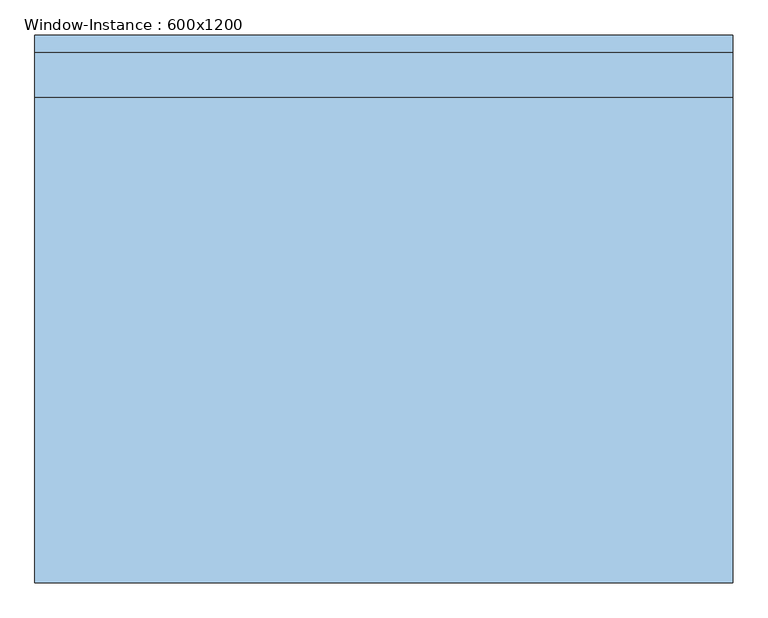
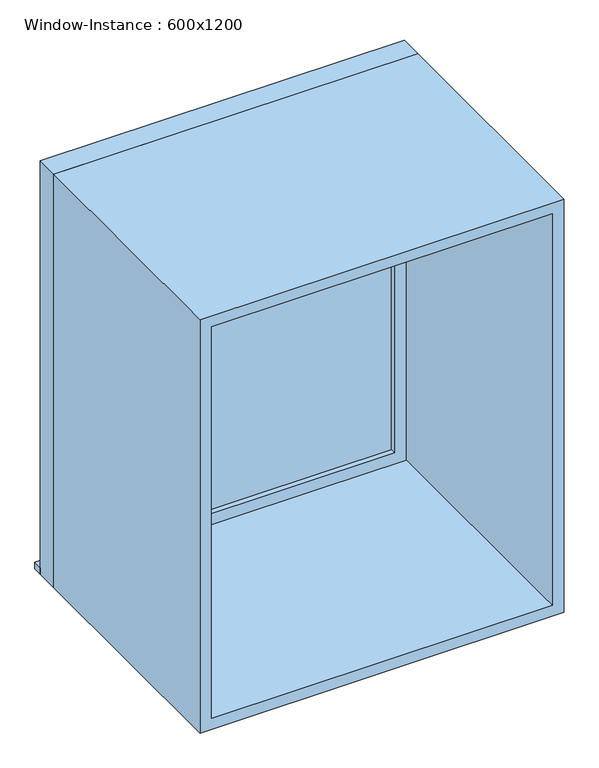
"""IFC4 building model written with IfcOpenShell, lengths in millimetres: window geometry, Window-Instance : 600x1200."""

from ifc_helpers import new_model, si_unit, frame, origin, place, context, project, spatial, polyline, outline, extrude, source, transform, mapped, element, save


def window_instance_600x1200_476e3a79(model_context):
    return source(origin(), model_context, "Body", "SweptSolid", [
        extrude(outline(polyline([(-538.1, 405.4), (461.9, 405.4), (461.9, 380.0), (-538.1, 380.0), (-538.1, 405.4)])), frame((0.0, 0.0, 900.0), z_axis=(0.0, 0.0, 1.0), x_axis=(1.0, 0.0, 0.0)), (0.0, 0.0, 1.0), 19.05),
        extrude(outline(polyline([(398.4, 331.425), (-474.6, 331.425), (-474.6, 344.125), (398.4, 344.125), (398.4, 331.425)])), frame((0.0, 0.0, 963.5), z_axis=(0.0, 0.0, 1.0), x_axis=(1.0, 0.0, 0.0)), (0.0, 0.0, 1.0), 1073.0),
        extrude(outline(polyline([(2080.95, -519.05), (919.05, -519.05), (919.05, 442.85), (2080.95, 442.85), (2080.95, -519.05)]), holes=[polyline([(2036.5, -474.6), (2036.5, 398.4), (963.5, 398.4), (963.5, -474.6), (2036.5, -474.6)])]), frame((0.0, 315.55, 0.0), z_axis=(0.0, 1.0, 0.0), x_axis=(0.0, 0.0, 1.0)), (0.0, 0.0, 1.0), 44.45),
        extrude(outline(polyline([(2100.0, -538.1), (900.0, -538.1), (900.0, 461.9), (2100.0, 461.9), (2100.0, -538.1)]), holes=[polyline([(2068.25, -506.35), (2068.25, 430.15), (931.75, 430.15), (931.75, -506.35), (2068.25, -506.35)])]), frame((0.0, -380.0, 0.0), z_axis=(0.0, 1.0, 0.0), x_axis=(0.0, 0.0, 1.0)), (0.0, 0.0, 1.0), 695.55),
        extrude(outline(polyline([(2100.0, 461.9), (2100.0, -538.1), (900.0, -538.1), (900.0, 461.9), (2100.0, 461.9)]), holes=[polyline([(2080.95, 442.85), (919.05, 442.85), (919.05, -519.05), (2080.95, -519.05), (2080.95, 442.85)])]), frame((0.0, 315.55, 0.0), z_axis=(0.0, 1.0, 0.0), x_axis=(0.0, 0.0, 1.0)), (0.0, 0.0, 1.0), 64.45),
    ])


if __name__ == "__main__":
    model = new_model("IFC4")
    model_context = context("Model", 3, world=origin())
    ifc_project = project(units=[si_unit("LENGTHUNIT", "METRE", prefix="MILLI")], contexts=[model_context])
    site = spatial("IfcSite", under=ifc_project)
    building = spatial("IfcBuilding", under=site)
    placement = place(None, origin())
    window_instance_600x1200_shape = window_instance_600x1200_476e3a79(model_context)
    element("IfcWindow", 1, ObjectType="Window-Instance : 600x1200", at=placement, inside=building, context=model_context, shape_type="MappedRepresentation", body=[
        mapped(window_instance_600x1200_shape, transform((0.0, 0.0, 0.0), x_axis=(1.0, 0.0, 0.0), y_axis=(0.0, 1.0, 0.0), z_axis=(0.0, 0.0, 1.0))),
    ])
    save(model, "model.ifc")

# Revit data of these elements
# Type "Window-Instance : 600x1200"
#   Type Mark = "7"
#   Construction Type Id = "GSP4R"
#   Assembly Code = "B2020100"
#   Analytic Construction = "1/8 in Pilkington single glazing"
#   Visual Light Transmittance = 0.9
#   Thermal Resistance (R) = 0.149095 (m²·K)/W
#   Solar Heat Gain Coefficient = 0.86
#   Heat Transfer Coefficient (U) = 6.70716 W/(m²·K)
#   Height [instance default] = 1200 mm
#   Default Sill Height = 900 mm
#   Width [instance default] = 600 mm
#   Window Inset = 20 mm
#   Glass Pane Material = WW-EC-GL-Storefront
#   Sash Material = WW-EC-RGB-White
#   Wall Closure = (empty or 0)
# Element 1 (IfcWindow, "Window-Instance : 600x1200")
#   Width = 1000 mm
#   Materials on its faces: "WW-EC-RGB-White", "WW-EC-GL-Storefront"
# Materials
#   "WW-EC-GL-Storefront": class "Glass", colour RGB 236 240 239, transparency 0.85, Description = "Storefront Glass", Cost = 0
#   "WW-EC-RGB-White": class "Generic", colour RGB 255 255 255, transparency 0, Comments = "If region requests off-white, swith asset color to RGB 231-228-220", Description = "Generic Color", Cost = 0
